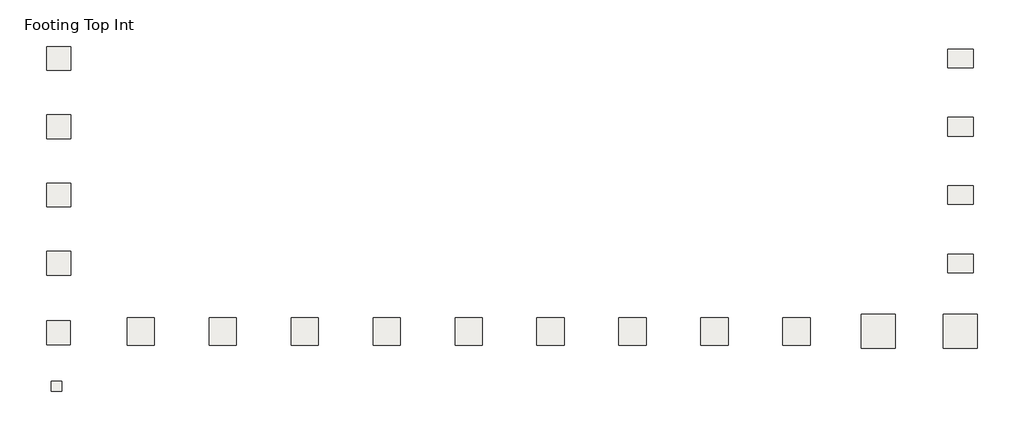
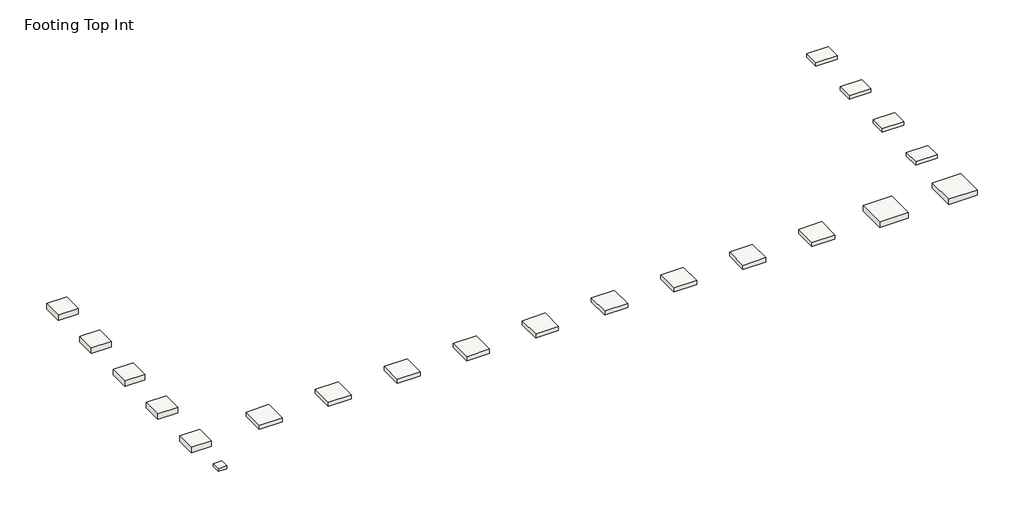
# One storey: 21 slabs.
"""IFC4 building model written with IfcOpenShell, lengths in millimetres."""

from ifc_helpers import new_model, si_unit, frame, origin, place, context, project, spatial, polyline, outline, extrude, element, save

model = new_model("IFC4")

# Units and contexts
model_context = context("Model", 3, world=origin())
ifc_project = project(units=[si_unit("LENGTHUNIT", "METRE", prefix="MILLI")], contexts=[model_context])

# Site, building, storey
site = spatial("IfcSite", under=ifc_project)
building = spatial("IfcBuilding", under=site)
storey = spatial("IfcBuildingStorey", under=building, Name="Footing Top Int", Elevation=-304.8)

# Slabs
placement = place(None, origin())
element("IfcSlab", 1, ObjectType="Footing-Rectangular : 36\" x 36\" x 12\"", at=placement, inside=storey, context=model_context, shape_type="SweptSolid", body=[
    extrude(outline(polyline([(323511.9648264, -572136.3413841), (323511.9648264, -573050.7413841), (322597.5648264, -573050.7413841), (322597.5648264, -572136.3413841), (323511.9648264, -572136.3413841)])), frame((0.0, 0.0, -609.6), z_axis=(0.0, 0.0, 1.0), x_axis=(1.0, 0.0, 0.0)), (0.0, 0.0, 1.0), 304.8),
])
element("IfcSlab", 2, ObjectType="Footing-Rectangular : 90\" x 66\" x 16\"", at=placement, inside=storey, context=model_context, shape_type="SweptSolid", body=[
    extrude(outline(polyline([(405277.7398264, -542342.1413841), (405277.7398264, -544018.5413841), (402991.7398264, -544018.5413841), (402991.7398264, -542342.1413841), (405277.7398264, -542342.1413841)])), frame((0.0, 0.0, -711.2), z_axis=(0.0, 0.0, 1.0), x_axis=(1.0, 0.0, 0.0)), (0.0, 0.0, 1.0), 406.4),
])
element("IfcSlab", 3, ObjectType="Footing-Rectangular : 90\" x 66\" x 16\"", at=placement, inside=storey, context=model_context, shape_type="SweptSolid", body=[
    extrude(outline(polyline([(405277.7398264, -548469.8913841), (405277.7398264, -550146.2913841), (402991.7398264, -550146.2913841), (402991.7398264, -548469.8913841), (405277.7398264, -548469.8913841)])), frame((0.0, 0.0, -711.2), z_axis=(0.0, 0.0, 1.0), x_axis=(1.0, 0.0, 0.0)), (0.0, 0.0, 1.0), 406.4),
])
element("IfcSlab", 4, ObjectType="Footing-Rectangular : 90\" x 66\" x 16\"", at=placement, inside=storey, context=model_context, shape_type="SweptSolid", body=[
    extrude(outline(polyline([(405277.7398264, -554597.6413841), (405277.7398264, -556274.0413841), (402991.7398264, -556274.0413841), (402991.7398264, -554597.6413841), (405277.7398264, -554597.6413841)])), frame((0.0, 0.0, -711.2), z_axis=(0.0, 0.0, 1.0), x_axis=(1.0, 0.0, 0.0)), (0.0, 0.0, 1.0), 406.4),
])
element("IfcSlab", 5, ObjectType="Footing-Rectangular : 90\" x 66\" x 16\"", at=placement, inside=storey, context=model_context, shape_type="SweptSolid", body=[
    extrude(outline(polyline([(405277.7398264, -560725.3913841), (405277.7398264, -562401.7913841), (402991.7398264, -562401.7913841), (402991.7398264, -560725.3913841), (405277.7398264, -560725.3913841)])), frame((0.0, 0.0, -711.2), z_axis=(0.0, 0.0, 1.0), x_axis=(1.0, 0.0, 0.0)), (0.0, 0.0, 1.0), 406.4),
])
element("IfcSlab", 6, ObjectType="Footing-Rectangular : F10", at=placement, inside=storey, context=model_context, shape_type="SweptSolid", body=[
    extrude(outline(polyline([(395257.4398264, -566141.9414082), (398305.4398264, -566141.9414082), (398305.4398264, -569189.9414082), (395257.4398264, -569189.9414082), (395257.4398264, -566141.9414082)])), frame((0.0, 0.0, -914.4), z_axis=(0.0, 0.0, 1.0), x_axis=(1.0, 0.0, 0.0)), (0.0, 0.0, 1.0), 609.6),
])
element("IfcSlab", 7, ObjectType="Footing-Rectangular : F10", at=placement, inside=storey, context=model_context, shape_type="SweptSolid", body=[
    extrude(outline(polyline([(402610.7398264, -566141.9414082), (405658.7398264, -566141.9414082), (405658.7398264, -569189.9414082), (402610.7398264, -569189.9414082), (402610.7398264, -566141.9414082)])), frame((0.0, 0.0, -914.4), z_axis=(0.0, 0.0, 1.0), x_axis=(1.0, 0.0, 0.0)), (0.0, 0.0, 1.0), 609.6),
])
element("IfcSlab", 8, ObjectType="Footing-Rectangular : F7", at=placement, inside=storey, context=model_context, shape_type="SweptSolid", body=[
    extrude(outline(polyline([(322156.2398264, -566707.0913841), (324289.8398264, -566707.0913841), (324289.8398264, -568840.6913841), (322156.2398264, -568840.6913841), (322156.2398264, -566707.0913841)])), frame((0.0, 0.0, -914.4), z_axis=(0.0, 0.0, 1.0), x_axis=(1.0, 0.0, 0.0)), (0.0, 0.0, 1.0), 609.6),
])
element("IfcSlab", 9, ObjectType="Footing-Rectangular : F7", at=placement, inside=storey, context=model_context, shape_type="SweptSolid", body=[
    extrude(outline(polyline([(324324.7648264, -542113.5413841), (324324.7648264, -544247.1413841), (322191.1648264, -544247.1413841), (322191.1648264, -542113.5413841), (324324.7648264, -542113.5413841)])), frame((0.0, 0.0, -914.4), z_axis=(0.0, 0.0, 1.0), x_axis=(1.0, 0.0, 0.0)), (0.0, 0.0, 1.0), 609.6),
])
element("IfcSlab", 10, ObjectType="Footing-Rectangular : F7", at=placement, inside=storey, context=model_context, shape_type="SweptSolid", body=[
    extrude(outline(polyline([(324324.7648264, -548241.2913841), (324324.7648264, -550374.8913841), (322191.1648264, -550374.8913841), (322191.1648264, -548241.2913841), (324324.7648264, -548241.2913841)])), frame((0.0, 0.0, -914.4), z_axis=(0.0, 0.0, 1.0), x_axis=(1.0, 0.0, 0.0)), (0.0, 0.0, 1.0), 609.6),
])
element("IfcSlab", 11, ObjectType="Footing-Rectangular : F7", at=placement, inside=storey, context=model_context, shape_type="SweptSolid", body=[
    extrude(outline(polyline([(324324.7648264, -554369.0413841), (324324.7648264, -556502.6413841), (322191.1648264, -556502.6413841), (322191.1648264, -554369.0413841), (324324.7648264, -554369.0413841)])), frame((0.0, 0.0, -914.4), z_axis=(0.0, 0.0, 1.0), x_axis=(1.0, 0.0, 0.0)), (0.0, 0.0, 1.0), 609.6),
])
element("IfcSlab", 12, ObjectType="Footing-Rectangular : F7", at=placement, inside=storey, context=model_context, shape_type="SweptSolid", body=[
    extrude(outline(polyline([(324324.7648264, -560496.7913841), (324324.7648264, -562630.3913841), (322191.1648264, -562630.3913841), (322191.1648264, -560496.7913841), (324324.7648264, -560496.7913841)])), frame((0.0, 0.0, -914.4), z_axis=(0.0, 0.0, 1.0), x_axis=(1.0, 0.0, 0.0)), (0.0, 0.0, 1.0), 609.6),
])
element("IfcSlab", 13, ObjectType="Footing-Rectangular : F8", at=placement, inside=storey, context=model_context, shape_type="SweptSolid", body=[
    extrude(outline(polyline([(329382.5398264, -566446.7414082), (331820.9398264, -566446.7414082), (331820.9398264, -568885.1414082), (329382.5398264, -568885.1414082), (329382.5398264, -566446.7414082)])), frame((0.0, 0.0, -762.0), z_axis=(0.0, 0.0, 1.0), x_axis=(1.0, 0.0, 0.0)), (0.0, 0.0, 1.0), 457.2),
])
element("IfcSlab", 14, ObjectType="Footing-Rectangular : F8", at=placement, inside=storey, context=model_context, shape_type="SweptSolid", body=[
    extrude(outline(polyline([(336735.8398264, -566446.7414082), (339174.2398264, -566446.7414082), (339174.2398264, -568885.1414082), (336735.8398264, -568885.1414082), (336735.8398264, -566446.7414082)])), frame((0.0, 0.0, -762.0), z_axis=(0.0, 0.0, 1.0), x_axis=(1.0, 0.0, 0.0)), (0.0, 0.0, 1.0), 457.2),
])
element("IfcSlab", 15, ObjectType="Footing-Rectangular : F8", at=placement, inside=storey, context=model_context, shape_type="SweptSolid", body=[
    extrude(outline(polyline([(344089.1398264, -566446.7414082), (346527.5398264, -566446.7414082), (346527.5398264, -568885.1414082), (344089.1398264, -568885.1414082), (344089.1398264, -566446.7414082)])), frame((0.0, 0.0, -762.0), z_axis=(0.0, 0.0, 1.0), x_axis=(1.0, 0.0, 0.0)), (0.0, 0.0, 1.0), 457.2),
])
element("IfcSlab", 16, ObjectType="Footing-Rectangular : F8", at=placement, inside=storey, context=model_context, shape_type="SweptSolid", body=[
    extrude(outline(polyline([(351442.4398264, -566446.7414082), (353880.8398264, -566446.7414082), (353880.8398264, -568885.1414082), (351442.4398264, -568885.1414082), (351442.4398264, -566446.7414082)])), frame((0.0, 0.0, -762.0), z_axis=(0.0, 0.0, 1.0), x_axis=(1.0, 0.0, 0.0)), (0.0, 0.0, 1.0), 457.2),
])
element("IfcSlab", 17, ObjectType="Footing-Rectangular : F8", at=placement, inside=storey, context=model_context, shape_type="SweptSolid", body=[
    extrude(outline(polyline([(358795.7398264, -566446.7414082), (361234.1398264, -566446.7414082), (361234.1398264, -568885.1414082), (358795.7398264, -568885.1414082), (358795.7398264, -566446.7414082)])), frame((0.0, 0.0, -762.0), z_axis=(0.0, 0.0, 1.0), x_axis=(1.0, 0.0, 0.0)), (0.0, 0.0, 1.0), 457.2),
])
element("IfcSlab", 18, ObjectType="Footing-Rectangular : F8", at=placement, inside=storey, context=model_context, shape_type="SweptSolid", body=[
    extrude(outline(polyline([(366149.0398264, -566446.7414082), (368587.4398264, -566446.7414082), (368587.4398264, -568885.1414082), (366149.0398264, -568885.1414082), (366149.0398264, -566446.7414082)])), frame((0.0, 0.0, -762.0), z_axis=(0.0, 0.0, 1.0), x_axis=(1.0, 0.0, 0.0)), (0.0, 0.0, 1.0), 457.2),
])
element("IfcSlab", 19, ObjectType="Footing-Rectangular : F8", at=placement, inside=storey, context=model_context, shape_type="SweptSolid", body=[
    extrude(outline(polyline([(373502.3398264, -566446.7414082), (375940.7398264, -566446.7414082), (375940.7398264, -568885.1414082), (373502.3398264, -568885.1414082), (373502.3398264, -566446.7414082)])), frame((0.0, 0.0, -762.0), z_axis=(0.0, 0.0, 1.0), x_axis=(1.0, 0.0, 0.0)), (0.0, 0.0, 1.0), 457.2),
])
element("IfcSlab", 20, ObjectType="Footing-Rectangular : F8", at=placement, inside=storey, context=model_context, shape_type="SweptSolid", body=[
    extrude(outline(polyline([(380855.6398264, -566446.7414082), (383294.0398264, -566446.7414082), (383294.0398264, -568885.1414082), (380855.6398264, -568885.1414082), (380855.6398264, -566446.7414082)])), frame((0.0, 0.0, -762.0), z_axis=(0.0, 0.0, 1.0), x_axis=(1.0, 0.0, 0.0)), (0.0, 0.0, 1.0), 457.2),
])
element("IfcSlab", 21, ObjectType="Footing-Rectangular : F8", at=placement, inside=storey, context=model_context, shape_type="SweptSolid", body=[
    extrude(outline(polyline([(388208.9398264, -566446.7414082), (390647.3398264, -566446.7414082), (390647.3398264, -568885.1414082), (388208.9398264, -568885.1414082), (388208.9398264, -566446.7414082)])), frame((0.0, 0.0, -762.0), z_axis=(0.0, 0.0, 1.0), x_axis=(1.0, 0.0, 0.0)), (0.0, 0.0, 1.0), 457.2),
])

save(model, "model.ifc")

# Revit data of these elements
# Type "Footing-Rectangular : 36\" x 36\" x 12\""
#   Assembly Code = "A1010100"
#   Width = 3' - 0"
#   Length = 3' - 0"
#   Thickness = 1' - 0"
#   Structural Material [instance default] = Concrete, Cast-in-Place gray
# Type "Footing-Rectangular : 90\" x 66\" x 16\""
#   Assembly Code = "A1010100"
#   Width = 7' - 6"
#   Length = 5' - 6"
#   Thickness = 1' - 4"
#   Structural Material [instance default] = Concrete, Cast-in-Place gray
# Type "Footing-Rectangular : F10"
#   Assembly Code = "A1010100"
#   Width = 10' - 0"
#   Length = 10' - 0"
#   Thickness = 2' - 0"
#   Structural Material [instance default] = Concrete, Cast-in-Place gray
# Type "Footing-Rectangular : F7"
#   Assembly Code = "A1010100"
#   Width = 7' - 0"
#   Length = 7' - 0"
#   Thickness = 2' - 0"
#   Structural Material [instance default] = Concrete, Cast-in-Place gray
# Type "Footing-Rectangular : F8"
#   Assembly Code = "A1010100"
#   Width = 8' - 0"
#   Length = 8' - 0"
#   Thickness = 1' - 6"
#   Structural Material [instance default] = Concrete, Cast-in-Place gray
# Element 1 (IfcSlab, "Footing-Rectangular : 36\" x 36\" x 12\"")
#   Comments = ""
#   Structural Material = Concrete, Cast-in-Place gray
#   Phase Created = New Construction
#   Materials on its faces: "Concrete, Cast-in-Place gray"
# Elements 2, 3, 4, 5 (IfcSlab, "Footing-Rectangular : 90\" x 66\" x 16\"")
#   Comments = ""
#   Structural Material = Concrete, Cast-in-Place gray
#   Phase Created = New Construction
#   Materials on its faces: "Concrete, Cast-in-Place gray"
# Elements 6, 7 (IfcSlab, "Footing-Rectangular : F10")
#   Comments = ""
#   Structural Material = Concrete, Cast-in-Place gray
#   Phase Created = New Construction
#   Materials on its faces: "Concrete, Cast-in-Place gray"
# Elements 8, 9, 10, 11, 12 (IfcSlab, "Footing-Rectangular : F7")
#   Comments = ""
#   Structural Material = Concrete, Cast-in-Place gray
#   Phase Created = New Construction
#   Materials on its faces: "Concrete, Cast-in-Place gray"
# Elements 13, 14, 15, 16, 17, 18, 19, 20, 21 (IfcSlab, "Footing-Rectangular : F8")
#   Comments = ""
#   Structural Material = Concrete, Cast-in-Place gray
#   Phase Created = New Construction
#   Materials on its faces: "Concrete, Cast-in-Place gray"
# Materials
#   "Concrete, Cast-in-Place gray": class "Concrete", colour RGB 192 192 192, transparency 0, Description = "Cast-in-place concrete", Cost = 0
